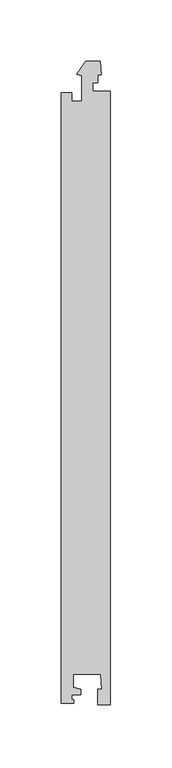
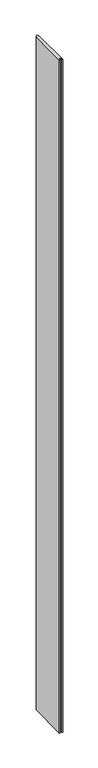
"""IFC4 building model written with IfcOpenShell, lengths in millimetres: proxy geometry, Generic Models 5:Generic Models 5:321804:Generic Models 5:321804 : Generic Models 5:Generic Models 5:321804:27 : Generic Models 5:Generic Models 5:321804:Generic Models 5:321804 : Generic Models 5:Generic Models 5:321804:300761."""

from ifc_helpers import new_model, si_unit, frame, origin, place, context, project, spatial, polyline, outline, extrude, source, transform, mapped, element, save


def generic_models_6a7d25ea(model_context):
    return source(origin(), model_context, "Body", "SweptSolid", [
        extrude(outline(polyline([(667625.2338797, -493910.833465), (667631.7338797, -493912.5751348), (667631.7338797, -493917.0251348), (667624.2338797, -493917.0251348), (667624.2338797, -493920.9751348), (667625.7338797, -493920.9751348), (667625.7338797, -493923.9751348), (667615.7338797, -493923.9751348), (667615.7338797, -493426.4751348), (667624.2338797, -493426.4751348), (667624.2338797, -493433.4251348), (667632.2338797, -493433.4251348), (667632.2338797, -493412.7091094), (667628.3059983, -493411.6566367), (667635.4133634, -493400.9751348), (667647.2715044, -493400.9751348), (667648.2338797, -493411.9751348), (667645.5338797, -493411.9751348), (667645.5338797, -493418.6001348), (667641.2338797, -493418.6001348), (667641.2338797, -493425.2251348), (667655.7338797, -493425.2251348), (667655.7338797, -493925.2251348), (667645.5338797, -493925.2251348), (667645.5338797, -493912.4751348), (667648.779534, -493912.4751348), (667647.72967, -493900.4751348), (667625.2338797, -493900.4751348), (667625.2338797, -493910.833465)])), frame((0.0, 0.0, -5.8417589), z_axis=(0.0, 0.0, 1.0), x_axis=(1.0, 0.0, 0.0)), (0.0, 0.0, 1.0), 8779.7126309),
    ])


if __name__ == "__main__":
    model = new_model("IFC4")
    model_context = context("Model", 3, world=origin())
    ifc_project = project(units=[si_unit("LENGTHUNIT", "METRE", prefix="MILLI")], contexts=[model_context])
    site = spatial("IfcSite", under=ifc_project)
    building = spatial("IfcBuilding", under=site)
    placement = place(None, origin())
    generic_models_shape = generic_models_6a7d25ea(model_context)
    element("IfcBuildingElementProxy", 1, Name="Generic Models 5:Generic Models 5:321804:Generic Models 5:321804 : Generic Models 5:Generic Models 5:321804:27 : Generic Models 5:Generic Models 5:321804:Generic Models 5:321804 : Generic Models 5:Generic Models 5:321804:300761", ObjectType="Generic Models 5:Generic Models 5:321804:Generic Models 5:321804 : Generic Models 5:Generic Models 5:321804:27 : Generic Models 5:Generic Models 5:321804:Generic Models 5:321804 : Generic Models 5:Generic Models 5:321804:300761", at=placement, inside=building, context=model_context, shape_type="MappedRepresentation", body=[
        mapped(generic_models_shape, transform((0.0, 0.0, 0.0), x_axis=(1.0, 0.0, 0.0), y_axis=(0.0, 1.0, 0.0), z_axis=(0.0, 0.0, 1.0))),
    ])
    save(model, "model.ifc")

# Revit data of these elements
# Type "Generic Models 5:Generic Models 5:321804:Generic Models 5:321804 : Generic Models 5:Generic Models 5:321804:27 : Generic Models 5:Generic Models 5:321804:Generic Models 5:321804 : Generic Models 5:Generic Models 5:321804:300761"
#   NameOverride = "Generic Models 5:Generic Models 5:321804:Generic Models 5:321804 : Generic Models 5:Generic Models 5:321804:300761"
#   ObjectTypeOverride = "Generic Models 5:321804 : Generic Models 5:Generic Models 5:321804"
#   Reference = "Generic Models 5"
#   Tag = "300761"
# Element 1 (IfcBuildingElementProxy, "Generic Models 5:Generic Models 5:321804:Generic Models 5:321804 : Generic Models 5:Generic Models 5:321804:27 : Generic Models 5:Generic Models 5:321804:Generic Models 5:321804 : Generic Models 5:Generic Models 5:321804:300761")
#   Materials on its faces: "POLYCARBONATE PANEL - ARCOPLUS 547"
# Materials
#   "POLYCARBONATE PANEL - ARCOPLUS 547": class "Unassigned", colour RGB 202 225 249, transparency 0.45, Cost = 0
